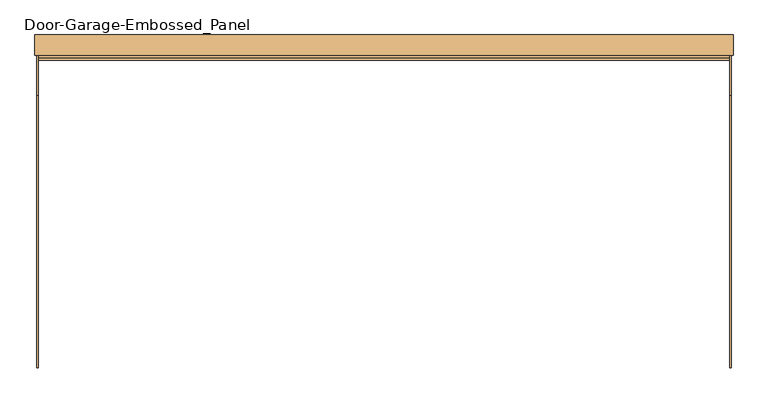
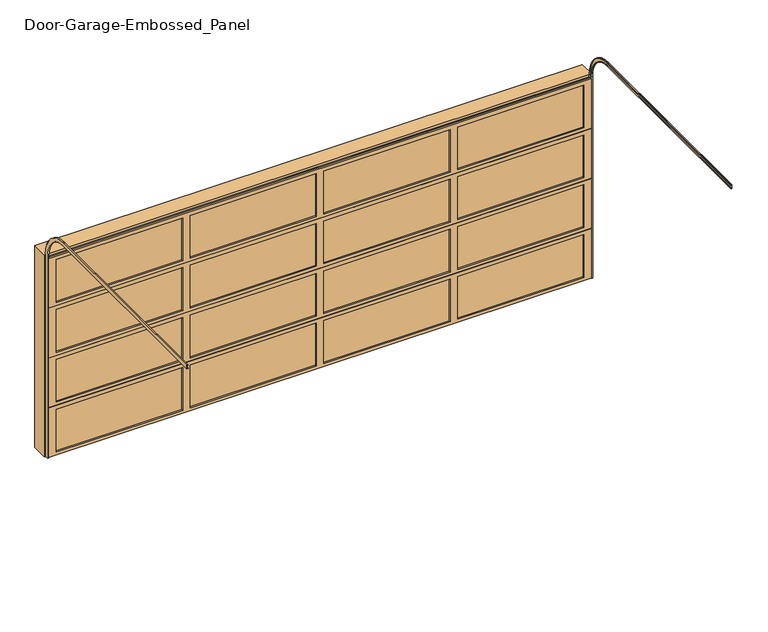
"""IFC4 building model written with IfcOpenShell, lengths in millimetres: door geometry, Door-Garage-Embossed_Panel : 216'' x 84''."""

from ifc_helpers import new_model, si_unit, frame, origin, place, context, project, spatial, polyline, circle_curve, outline, extrude, faceted_brep, source, transform, mapped, element, save
from ifc_brep_helpers import plane_surface, cylinder_surface, revolved_surface, advanced_brep


def door_garage_embossed_panel_c404131a(model_context):
    return source(origin(), model_context, "Body", "SolidModel", [
        extrude(outline(polyline([(1314.45, -100.0125), (1314.45, -106.3625), (38.1, -106.3625), (38.1, -100.0125), (1314.45, -100.0125)])), frame((0.0, 0.0, 1638.3), z_axis=(0.0, 0.0, 1.0), x_axis=(1.0, 0.0, 0.0)), (0.0, 0.0, 1.0), 457.2),
        extrude(outline(polyline([(-38.1, -100.0125), (-38.1, -106.3625), (-1314.45, -106.3625), (-1314.45, -100.0125), (-38.1, -100.0125)])), frame((0.0, 0.0, 1638.3), z_axis=(0.0, 0.0, 1.0), x_axis=(1.0, 0.0, 0.0)), (0.0, 0.0, 1.0), 457.2),
        extrude(outline(polyline([(2667.0, -100.0125), (2667.0, -106.3625), (1390.65, -106.3625), (1390.65, -100.0125), (2667.0, -100.0125)])), frame((0.0, 0.0, 1638.3), z_axis=(0.0, 0.0, 1.0), x_axis=(1.0, 0.0, 0.0)), (0.0, 0.0, 1.0), 457.2),
        extrude(outline(polyline([(-1390.65, -100.0125), (-1390.65, -106.3625), (-2667.0, -106.3625), (-2667.0, -100.0125), (-1390.65, -100.0125)])), frame((0.0, 0.0, 1638.3), z_axis=(0.0, 0.0, 1.0), x_axis=(1.0, 0.0, 0.0)), (0.0, 0.0, 1.0), 457.2),
        faceted_brep([(2743.2, -106.3625, 2136.775), (2743.2, -122.2375, 2136.775), (2743.2, -122.2375, 1606.55), (2743.2, -100.0125, 1606.55), (2743.2, -100.0125, 1600.2), (2743.2, -84.1375, 1600.2), (2743.2, -84.1375, 2130.425), (2743.2, -106.3625, 2130.425), (-2743.2, -122.2375, 2136.775), (-2743.2, -106.3625, 2136.775), (-2743.2, -106.3625, 2130.425), (-2743.2, -84.1375, 2130.425), (-2743.2, -84.1375, 1600.2), (-2743.2, -100.0125, 1600.2), (-2743.2, -100.0125, 1606.55), (-2743.2, -122.2375, 1606.55), (1390.65, -122.2375, 2095.5), (2667.0, -122.2375, 2095.5), (2667.0, -122.2375, 1638.3), (1390.65, -122.2375, 1638.3), (-1314.45, -122.2375, 2095.5), (-38.1, -122.2375, 2095.5), (-38.1, -122.2375, 1638.3), (-1314.45, -122.2375, 1638.3), (38.1, -122.2375, 2095.5), (1314.45, -122.2375, 2095.5), (1314.45, -122.2375, 1638.3), (38.1, -122.2375, 1638.3), (-2667.0, -122.2375, 2095.5), (-1390.65, -122.2375, 2095.5), (-1390.65, -122.2375, 1638.3), (-2667.0, -122.2375, 1638.3), (2667.0, -84.1375, 2095.5), (1390.65, -84.1375, 2095.5), (1390.65, -84.1375, 1638.3), (2667.0, -84.1375, 1638.3), (-38.1, -84.1375, 2095.5), (-1314.45, -84.1375, 2095.5), (-1314.45, -84.1375, 1638.3), (-38.1, -84.1375, 1638.3), (1314.45, -84.1375, 2095.5), (38.1, -84.1375, 2095.5), (38.1, -84.1375, 1638.3), (1314.45, -84.1375, 1638.3), (-1390.65, -84.1375, 2095.5), (-2667.0, -84.1375, 2095.5), (-2667.0, -84.1375, 1638.3), (-1390.65, -84.1375, 1638.3)], [[[0, 1, 2, 3, 4, 5, 6, 7]], [[8, 9, 10, 11, 12, 13, 14, 15]], [[1, 0, 9, 8]], [[2, 1, 8, 15], [16, 17, 18, 19], [20, 21, 22, 23], [24, 25, 26, 27], [28, 29, 30, 31]], [[3, 2, 15, 14]], [[4, 3, 14, 13]], [[5, 4, 13, 12]], [[6, 5, 12, 11], [32, 33, 34, 35], [36, 37, 38, 39], [40, 41, 42, 43], [44, 45, 46, 47]], [[7, 6, 11, 10]], [[0, 7, 10, 9]], [[16, 33, 32, 17]], [[33, 16, 19, 34]], [[34, 19, 18, 35]], [[17, 32, 35, 18]], [[20, 37, 36, 21]], [[37, 20, 23, 38]], [[38, 23, 22, 39]], [[21, 36, 39, 22]], [[24, 41, 40, 25]], [[41, 24, 27, 42]], [[42, 27, 26, 43]], [[25, 40, 43, 26]], [[28, 45, 44, 29]], [[45, 28, 31, 46]], [[46, 31, 30, 47]], [[29, 44, 47, 30]]]),
        extrude(outline(polyline([(1314.45, -100.0125), (1314.45, -106.3625), (38.1, -106.3625), (38.1, -100.0125), (1314.45, -100.0125)])), frame((0.0, 0.0, 1104.9), z_axis=(0.0, 0.0, 1.0), x_axis=(1.0, 0.0, 0.0)), (0.0, 0.0, 1.0), 457.2),
        extrude(outline(polyline([(-38.1, -100.0125), (-38.1, -106.3625), (-1314.45, -106.3625), (-1314.45, -100.0125), (-38.1, -100.0125)])), frame((0.0, 0.0, 1104.9), z_axis=(0.0, 0.0, 1.0), x_axis=(1.0, 0.0, 0.0)), (0.0, 0.0, 1.0), 457.2),
        extrude(outline(polyline([(2667.0, -100.0125), (2667.0, -106.3625), (1390.65, -106.3625), (1390.65, -100.0125), (2667.0, -100.0125)])), frame((0.0, 0.0, 1104.9), z_axis=(0.0, 0.0, 1.0), x_axis=(1.0, 0.0, 0.0)), (0.0, 0.0, 1.0), 457.2),
        extrude(outline(polyline([(-1390.65, -100.0125), (-1390.65, -106.3625), (-2667.0, -106.3625), (-2667.0, -100.0125), (-1390.65, -100.0125)])), frame((0.0, 0.0, 1104.9), z_axis=(0.0, 0.0, 1.0), x_axis=(1.0, 0.0, 0.0)), (0.0, 0.0, 1.0), 457.2),
        faceted_brep([(2743.2, -106.3625, 1603.375), (2743.2, -122.2375, 1603.375), (2743.2, -122.2375, 1073.15), (2743.2, -100.0125, 1073.15), (2743.2, -100.0125, 1066.8), (2743.2, -84.1375, 1066.8), (2743.2, -84.1375, 1597.025), (2743.2, -106.3625, 1597.025), (-2743.2, -122.2375, 1603.375), (-2743.2, -106.3625, 1603.375), (-2743.2, -106.3625, 1597.025), (-2743.2, -84.1375, 1597.025), (-2743.2, -84.1375, 1066.8), (-2743.2, -100.0125, 1066.8), (-2743.2, -100.0125, 1073.15), (-2743.2, -122.2375, 1073.15), (1390.65, -122.2375, 1562.1), (2667.0, -122.2375, 1562.1), (2667.0, -122.2375, 1104.9), (1390.65, -122.2375, 1104.9), (-1314.45, -122.2375, 1562.1), (-38.1, -122.2375, 1562.1), (-38.1, -122.2375, 1104.9), (-1314.45, -122.2375, 1104.9), (38.1, -122.2375, 1562.1), (1314.45, -122.2375, 1562.1), (1314.45, -122.2375, 1104.9), (38.1, -122.2375, 1104.9), (-2667.0, -122.2375, 1562.1), (-1390.65, -122.2375, 1562.1), (-1390.65, -122.2375, 1104.9), (-2667.0, -122.2375, 1104.9), (2667.0, -84.1375, 1562.1), (1390.65, -84.1375, 1562.1), (1390.65, -84.1375, 1104.9), (2667.0, -84.1375, 1104.9), (-38.1, -84.1375, 1562.1), (-1314.45, -84.1375, 1562.1), (-1314.45, -84.1375, 1104.9), (-38.1, -84.1375, 1104.9), (1314.45, -84.1375, 1562.1), (38.1, -84.1375, 1562.1), (38.1, -84.1375, 1104.9), (1314.45, -84.1375, 1104.9), (-1390.65, -84.1375, 1562.1), (-2667.0, -84.1375, 1562.1), (-2667.0, -84.1375, 1104.9), (-1390.65, -84.1375, 1104.9)], [[[0, 1, 2, 3, 4, 5, 6, 7]], [[8, 9, 10, 11, 12, 13, 14, 15]], [[1, 0, 9, 8]], [[2, 1, 8, 15], [16, 17, 18, 19], [20, 21, 22, 23], [24, 25, 26, 27], [28, 29, 30, 31]], [[3, 2, 15, 14]], [[4, 3, 14, 13]], [[5, 4, 13, 12]], [[6, 5, 12, 11], [32, 33, 34, 35], [36, 37, 38, 39], [40, 41, 42, 43], [44, 45, 46, 47]], [[7, 6, 11, 10]], [[0, 7, 10, 9]], [[16, 33, 32, 17]], [[33, 16, 19, 34]], [[34, 19, 18, 35]], [[17, 32, 35, 18]], [[20, 37, 36, 21]], [[37, 20, 23, 38]], [[38, 23, 22, 39]], [[21, 36, 39, 22]], [[24, 41, 40, 25]], [[41, 24, 27, 42]], [[42, 27, 26, 43]], [[25, 40, 43, 26]], [[28, 45, 44, 29]], [[45, 28, 31, 46]], [[46, 31, 30, 47]], [[29, 44, 47, 30]]]),
        extrude(outline(polyline([(1314.45, -100.0125), (1314.45, -106.3625), (38.1, -106.3625), (38.1, -100.0125), (1314.45, -100.0125)])), frame((0.0, 0.0, 571.5), z_axis=(0.0, 0.0, 1.0), x_axis=(1.0, 0.0, 0.0)), (0.0, 0.0, 1.0), 457.2),
        extrude(outline(polyline([(-38.1, -100.0125), (-38.1, -106.3625), (-1314.45, -106.3625), (-1314.45, -100.0125), (-38.1, -100.0125)])), frame((0.0, 0.0, 571.5), z_axis=(0.0, 0.0, 1.0), x_axis=(1.0, 0.0, 0.0)), (0.0, 0.0, 1.0), 457.2),
        extrude(outline(polyline([(2667.0, -100.0125), (2667.0, -106.3625), (1390.65, -106.3625), (1390.65, -100.0125), (2667.0, -100.0125)])), frame((0.0, 0.0, 571.5), z_axis=(0.0, 0.0, 1.0), x_axis=(1.0, 0.0, 0.0)), (0.0, 0.0, 1.0), 457.2),
        extrude(outline(polyline([(-1390.65, -100.0125), (-1390.65, -106.3625), (-2667.0, -106.3625), (-2667.0, -100.0125), (-1390.65, -100.0125)])), frame((0.0, 0.0, 571.5), z_axis=(0.0, 0.0, 1.0), x_axis=(1.0, 0.0, 0.0)), (0.0, 0.0, 1.0), 457.2),
        faceted_brep([(2743.2, -106.3625, 1069.975), (2743.2, -122.2375, 1069.975), (2743.2, -122.2375, 539.75), (2743.2, -100.0125, 539.75), (2743.2, -100.0125, 533.4), (2743.2, -84.1375, 533.4), (2743.2, -84.1375, 1063.625), (2743.2, -106.3625, 1063.625), (-2743.2, -122.2375, 1069.975), (-2743.2, -106.3625, 1069.975), (-2743.2, -106.3625, 1063.625), (-2743.2, -84.1375, 1063.625), (-2743.2, -84.1375, 533.4), (-2743.2, -100.0125, 533.4), (-2743.2, -100.0125, 539.75), (-2743.2, -122.2375, 539.75), (1390.65, -122.2375, 1028.7), (2667.0, -122.2375, 1028.7), (2667.0, -122.2375, 571.5), (1390.65, -122.2375, 571.5), (-1314.45, -122.2375, 1028.7), (-38.1, -122.2375, 1028.7), (-38.1, -122.2375, 571.5), (-1314.45, -122.2375, 571.5), (38.1, -122.2375, 1028.7), (1314.45, -122.2375, 1028.7), (1314.45, -122.2375, 571.5), (38.1, -122.2375, 571.5), (-2667.0, -122.2375, 1028.7), (-1390.65, -122.2375, 1028.7), (-1390.65, -122.2375, 571.5), (-2667.0, -122.2375, 571.5), (2667.0, -84.1375, 1028.7), (1390.65, -84.1375, 1028.7), (1390.65, -84.1375, 571.5), (2667.0, -84.1375, 571.5), (-38.1, -84.1375, 1028.7), (-1314.45, -84.1375, 1028.7), (-1314.45, -84.1375, 571.5), (-38.1, -84.1375, 571.5), (1314.45, -84.1375, 1028.7), (38.1, -84.1375, 1028.7), (38.1, -84.1375, 571.5), (1314.45, -84.1375, 571.5), (-1390.65, -84.1375, 1028.7), (-2667.0, -84.1375, 1028.7), (-2667.0, -84.1375, 571.5), (-1390.65, -84.1375, 571.5)], [[[0, 1, 2, 3, 4, 5, 6, 7]], [[8, 9, 10, 11, 12, 13, 14, 15]], [[1, 0, 9, 8]], [[2, 1, 8, 15], [16, 17, 18, 19], [20, 21, 22, 23], [24, 25, 26, 27], [28, 29, 30, 31]], [[3, 2, 15, 14]], [[4, 3, 14, 13]], [[5, 4, 13, 12]], [[6, 5, 12, 11], [32, 33, 34, 35], [36, 37, 38, 39], [40, 41, 42, 43], [44, 45, 46, 47]], [[7, 6, 11, 10]], [[0, 7, 10, 9]], [[16, 33, 32, 17]], [[33, 16, 19, 34]], [[34, 19, 18, 35]], [[17, 32, 35, 18]], [[20, 37, 36, 21]], [[37, 20, 23, 38]], [[38, 23, 22, 39]], [[21, 36, 39, 22]], [[24, 41, 40, 25]], [[41, 24, 27, 42]], [[42, 27, 26, 43]], [[25, 40, 43, 26]], [[28, 45, 44, 29]], [[45, 28, 31, 46]], [[46, 31, 30, 47]], [[29, 44, 47, 30]]]),
        extrude(outline(polyline([(1314.45, -100.0125), (1314.45, -106.3625), (38.1, -106.3625), (38.1, -100.0125), (1314.45, -100.0125)])), frame((0.0, 0.0, 38.1), z_axis=(0.0, 0.0, 1.0), x_axis=(1.0, 0.0, 0.0)), (0.0, 0.0, 1.0), 457.2),
        extrude(outline(polyline([(-38.1, -100.0125), (-38.1, -106.3625), (-1314.45, -106.3625), (-1314.45, -100.0125), (-38.1, -100.0125)])), frame((0.0, 0.0, 38.1), z_axis=(0.0, 0.0, 1.0), x_axis=(1.0, 0.0, 0.0)), (0.0, 0.0, 1.0), 457.2),
        extrude(outline(polyline([(2667.0, -100.0125), (2667.0, -106.3625), (1390.65, -106.3625), (1390.65, -100.0125), (2667.0, -100.0125)])), frame((0.0, 0.0, 38.1), z_axis=(0.0, 0.0, 1.0), x_axis=(1.0, 0.0, 0.0)), (0.0, 0.0, 1.0), 457.2),
        extrude(outline(polyline([(-1390.65, -100.0125), (-1390.65, -106.3625), (-2667.0, -106.3625), (-2667.0, -100.0125), (-1390.65, -100.0125)])), frame((0.0, 0.0, 38.1), z_axis=(0.0, 0.0, 1.0), x_axis=(1.0, 0.0, 0.0)), (0.0, 0.0, 1.0), 457.2),
        faceted_brep([(2743.2, -106.3625, 536.575), (2743.2, -122.2375, 536.575), (2743.2, -122.2375, 6.35), (2743.2, -100.0125, 6.35), (2743.2, -100.0125, 0.0), (2743.2, -84.1375, 0.0), (2743.2, -84.1375, 530.225), (2743.2, -106.3625, 530.225), (-2743.2, -122.2375, 536.575), (-2743.2, -106.3625, 536.575), (-2743.2, -106.3625, 530.225), (-2743.2, -84.1375, 530.225), (-2743.2, -84.1375, 0.0), (-2743.2, -100.0125, 0.0), (-2743.2, -100.0125, 6.35), (-2743.2, -122.2375, 6.35), (1390.65, -122.2375, 495.3), (2667.0, -122.2375, 495.3), (2667.0, -122.2375, 38.1), (1390.65, -122.2375, 38.1), (-1314.45, -122.2375, 495.3), (-38.1, -122.2375, 495.3), (-38.1, -122.2375, 38.1), (-1314.45, -122.2375, 38.1), (38.1, -122.2375, 495.3), (1314.45, -122.2375, 495.3), (1314.45, -122.2375, 38.1), (38.1, -122.2375, 38.1), (-2667.0, -122.2375, 495.3), (-1390.65, -122.2375, 495.3), (-1390.65, -122.2375, 38.1), (-2667.0, -122.2375, 38.1), (2667.0, -84.1375, 495.3), (1390.65, -84.1375, 495.3), (1390.65, -84.1375, 38.1), (2667.0, -84.1375, 38.1), (-38.1, -84.1375, 495.3), (-1314.45, -84.1375, 495.3), (-1314.45, -84.1375, 38.1), (-38.1, -84.1375, 38.1), (1314.45, -84.1375, 495.3), (38.1, -84.1375, 495.3), (38.1, -84.1375, 38.1), (1314.45, -84.1375, 38.1), (-1390.65, -84.1375, 495.3), (-2667.0, -84.1375, 495.3), (-2667.0, -84.1375, 38.1), (-1390.65, -84.1375, 38.1)], [[[0, 1, 2, 3, 4, 5, 6, 7]], [[8, 9, 10, 11, 12, 13, 14, 15]], [[1, 0, 9, 8]], [[2, 1, 8, 15], [16, 17, 18, 19], [20, 21, 22, 23], [24, 25, 26, 27], [28, 29, 30, 31]], [[3, 2, 15, 14]], [[4, 3, 14, 13]], [[5, 4, 13, 12]], [[6, 5, 12, 11], [32, 33, 34, 35], [36, 37, 38, 39], [40, 41, 42, 43], [44, 45, 46, 47]], [[7, 6, 11, 10]], [[0, 7, 10, 9]], [[16, 33, 32, 17]], [[33, 16, 19, 34]], [[34, 19, 18, 35]], [[17, 32, 35, 18]], [[20, 37, 36, 21]], [[37, 20, 23, 38]], [[38, 23, 22, 39]], [[21, 36, 39, 22]], [[24, 41, 40, 25]], [[41, 24, 27, 42]], [[42, 27, 26, 43]], [[25, 40, 43, 26]], [[28, 45, 44, 29]], [[45, 28, 31, 46]], [[46, 31, 30, 47]], [[29, 44, 47, 30]]]),
        advanced_brep(
        [(2755.9, -122.2375, 0.0), (2743.2, -122.2375, 0.0), (2743.2, -119.0625, 0.0), (2752.725, -119.0625, 0.0), (2752.725, -87.3125, 0.0), (2743.2, -87.3125, 0.0), (2743.2, -84.1375, 0.0), (2755.9, -84.1375, 0.0), (2755.9, -122.2375, 2159.0), (2743.2, -122.2375, 2159.0), (2743.2, -401.6375, 2438.4), (2743.2, -2560.6375, 2438.4), (2743.2, -2560.6375, 2441.575), (2743.2, -401.6375, 2441.575), (2743.2, -119.0625, 2159.0), (2752.725, -119.0625, 2159.0), (2752.725, -401.6375, 2441.575), (2752.725, -2560.6375, 2441.575), (2752.725, -2560.6375, 2473.325), (2752.725, -401.6375, 2473.325), (2752.725, -87.3125, 2159.0), (2743.2, -87.3125, 2159.0), (2743.2, -401.6375, 2473.325), (2743.2, -2560.6375, 2473.325), (2743.2, -2560.6375, 2476.5), (2743.2, -401.6375, 2476.5), (2743.2, -84.1375, 2159.0), (2755.9, -84.1375, 2159.0), (2755.9, -401.6375, 2476.5), (2755.9, -2560.6375, 2476.5), (2755.9, -2560.6375, 2438.4), (2755.9, -401.6375, 2438.4)],
        [
            (0, 1),
            (1, 2),
            (2, 3),
            (3, 4),
            (4, 5),
            (5, 6),
            (6, 7),
            (7, 0),
            (0, 8),
            (8, 9),
            (9, 1),
            (9, 10, circle_curve(frame((2743.2, -401.6375, 2159.0), z_axis=(1.0, 0.0, 0.0), x_axis=(0.0, 1.0, 0.0)), 279.4)),
            (10, 11),
            (11, 12),
            (12, 13),
            (13, 14, circle_curve(frame((2743.2, -401.6375, 2159.0), z_axis=(-1.0, 0.0, 0.0), x_axis=(0.0, 1.0, 0.0)), 282.575)),
            (14, 2),
            (14, 15),
            (15, 3),
            (15, 16, circle_curve(frame((2752.725, -401.6375, 2159.0), z_axis=(1.0, 0.0, 0.0), x_axis=(0.0, 1.0, 0.0)), 282.575)),
            (16, 17),
            (17, 18),
            (18, 19),
            (19, 20, circle_curve(frame((2752.725, -401.6375, 2159.0), z_axis=(-1.0, 0.0, 0.0), x_axis=(0.0, 1.0, 0.0)), 314.325)),
            (20, 4),
            (20, 21),
            (21, 5),
            (21, 22, circle_curve(frame((2743.2, -401.6375, 2159.0), z_axis=(1.0, 0.0, 0.0), x_axis=(0.0, 1.0, 0.0)), 314.325)),
            (22, 23),
            (23, 24),
            (24, 25),
            (25, 26, circle_curve(frame((2743.2, -401.6375, 2159.0), z_axis=(-1.0, 0.0, 0.0), x_axis=(0.0, 1.0, 0.0)), 317.5)),
            (26, 6),
            (26, 27),
            (27, 7),
            (27, 28, circle_curve(frame((2755.9, -401.6375, 2159.0), z_axis=(1.0, 0.0, 0.0), x_axis=(0.0, 1.0, 0.0)), 317.5)),
            (28, 29),
            (29, 30),
            (30, 31),
            (31, 8, circle_curve(frame((2755.9, -401.6375, 2159.0), z_axis=(-1.0, 0.0, 0.0), x_axis=(0.0, 1.0, 0.0)), 279.4)),
            (31, 10),
            (13, 16),
            (19, 22),
            (25, 28),
            (29, 24),
            (23, 18),
            (17, 12),
            (11, 30),
        ],
        [
            plane_surface(frame((0.0, -122.2375, 0.0), z_axis=(0.0, 0.0, -1.0), x_axis=(1.0, 0.0, 0.0))),
            plane_surface(frame((2755.9, -122.2375, 0.0), z_axis=(0.0, -1.0, 0.0), x_axis=(0.0, 0.0, 1.0))),
            plane_surface(frame((2743.2, -122.2375, 0.0), z_axis=(-1.0, 0.0, 0.0), x_axis=(0.0, 0.0, 1.0))),
            plane_surface(frame((2743.2, -119.0625, 0.0), z_axis=(0.0, 1.0, 0.0), x_axis=(0.0, 0.0, 1.0))),
            plane_surface(frame((2752.725, -119.0625, 0.0), z_axis=(-1.0, 0.0, 0.0), x_axis=(0.0, 0.0, 1.0))),
            plane_surface(frame((2752.725, -87.3125, 0.0), z_axis=(0.0, -1.0, 0.0), x_axis=(0.0, 0.0, 1.0))),
            plane_surface(frame((2743.2, -87.3125, 0.0), z_axis=(-1.0, 0.0, 0.0), x_axis=(0.0, 0.0, 1.0))),
            plane_surface(frame((2743.2, -84.1375, 0.0), z_axis=(0.0, 1.0, 0.0), x_axis=(0.0, 0.0, 1.0))),
            plane_surface(frame((2755.9, -84.1375, 0.0), z_axis=(1.0, 0.0, 0.0), x_axis=(0.0, 0.0, 1.0))),
            revolved_surface(polyline([(2755.9, -122.23750000000001, 2159.0), (2743.2, -122.23750000000001, 2159.0)]), (0.0, -401.6375, 2159.0), (1.0, 0.0, 0.0)),
            cylinder_surface(frame((0.0, -401.6375, 2159.0), z_axis=(1.0, 0.0, 0.0), x_axis=(0.0, 1.0, 0.0)), 282.575),
            revolved_surface(polyline([(2752.725, -87.3125, 2159.0), (2743.2, -87.3125, 2159.0)]), (0.0, -401.6375, 2159.0), (1.0, 0.0, 0.0)),
            cylinder_surface(frame((0.0, -401.6375, 2159.0), z_axis=(1.0, 0.0, 0.0), x_axis=(0.0, 1.0, 0.0)), 317.5),
            plane_surface(frame((0.0, -2560.6375, 2438.4), z_axis=(0.0, -1.0, 0.0), x_axis=(1.0, 0.0, 0.0))),
            plane_surface(frame((2755.9, -401.6375, 2438.4), z_axis=(0.0, 0.0, -1.0), x_axis=(0.0, -1.0, 0.0))),
            plane_surface(frame((2743.2, -401.6375, 2441.575), z_axis=(0.0, 0.0, 1.0), x_axis=(0.0, -1.0, 0.0))),
            plane_surface(frame((2752.725, -401.6375, 2473.325), z_axis=(0.0, 0.0, -1.0), x_axis=(0.0, -1.0, 0.0))),
            plane_surface(frame((2743.2, -401.6375, 2476.5), z_axis=(0.0, 0.0, 1.0), x_axis=(0.0, -1.0, 0.0))),
        ],
        [
            (0, [[1, 2, 3, 4, 5, 6, 7, 8]]),
            (1, [[-1, 9, 10, 11]]),
            (2, [[-2, -11, 12, 13, 14, 15, 16, 17]]),
            (3, [[-3, -17, 18, 19]]),
            (4, [[-4, -19, 20, 21, 22, 23, 24, 25]]),
            (5, [[-5, -25, 26, 27]]),
            (6, [[-6, -27, 28, 29, 30, 31, 32, 33]]),
            (7, [[-7, -33, 34, 35]]),
            (8, [[-8, -35, 36, 37, 38, 39, 40, -9]]),
            (9, [[-12, -10, -40, 41]]),
            (10, [[-20, -18, -16, 42]]),
            (11, [[-28, -26, -24, 43]]),
            (12, [[-36, -34, -32, 44]]),
            (13, [[-38, 45, -30, 46, -22, 47, -14, 48]]),
            (14, [[-41, -39, -48, -13]]),
            (15, [[-42, -15, -47, -21]]),
            (16, [[-43, -23, -46, -29]]),
            (17, [[-44, -31, -45, -37]]),
        ],
    ),
        advanced_brep(
        [(-2755.9, -122.2375, 0.0), (-2755.9, -84.1375, 0.0), (-2743.2, -84.1375, 0.0), (-2743.2, -87.3125, 0.0), (-2752.725, -87.3125, 0.0), (-2752.725, -119.0625, 0.0), (-2743.2, -119.0625, 0.0), (-2743.2, -122.2375, 0.0), (-2755.9, -122.2375, 2159.0), (-2755.9, -401.6375, 2438.4), (-2755.9, -2560.6375, 2438.4), (-2755.9, -2560.6375, 2476.5), (-2755.9, -401.6375, 2476.5), (-2755.9, -84.1375, 2159.0), (-2743.2, -84.1375, 2159.0), (-2743.2, -401.6375, 2476.5), (-2743.2, -2560.6375, 2476.5), (-2743.2, -2560.6375, 2473.325), (-2743.2, -401.6375, 2473.325), (-2743.2, -87.3125, 2159.0), (-2752.725, -87.3125, 2159.0), (-2752.725, -401.6375, 2473.325), (-2752.725, -2560.6375, 2473.325), (-2752.725, -2560.6375, 2441.575), (-2752.725, -401.6375, 2441.575), (-2752.725, -119.0625, 2159.0), (-2743.2, -119.0625, 2159.0), (-2743.2, -401.6375, 2441.575), (-2743.2, -2560.6375, 2441.575), (-2743.2, -2560.6375, 2438.4), (-2743.2, -401.6375, 2438.4), (-2743.2, -122.2375, 2159.0)],
        [
            (0, 1),
            (1, 2),
            (2, 3),
            (3, 4),
            (4, 5),
            (5, 6),
            (6, 7),
            (7, 0),
            (0, 8),
            (8, 9, circle_curve(frame((-2755.9, -401.6375, 2159.0), z_axis=(1.0, 0.0, 0.0), x_axis=(0.0, 1.0, 0.0)), 279.4)),
            (9, 10),
            (10, 11),
            (11, 12),
            (12, 13, circle_curve(frame((-2755.9, -401.6375, 2159.0), z_axis=(-1.0, 0.0, 0.0), x_axis=(0.0, 1.0, 0.0)), 317.5)),
            (13, 1),
            (13, 14),
            (14, 2),
            (14, 15, circle_curve(frame((-2743.2, -401.6375, 2159.0), z_axis=(1.0, 0.0, 0.0), x_axis=(0.0, 1.0, 0.0)), 317.5)),
            (15, 16),
            (16, 17),
            (17, 18),
            (18, 19, circle_curve(frame((-2743.2, -401.6375, 2159.0), z_axis=(-1.0, 0.0, 0.0), x_axis=(0.0, 1.0, 0.0)), 314.325)),
            (19, 3),
            (19, 20),
            (20, 4),
            (20, 21, circle_curve(frame((-2752.725, -401.6375, 2159.0), z_axis=(1.0, 0.0, 0.0), x_axis=(0.0, 1.0, 0.0)), 314.325)),
            (21, 22),
            (22, 23),
            (23, 24),
            (24, 25, circle_curve(frame((-2752.725, -401.6375, 2159.0), z_axis=(-1.0, 0.0, 0.0), x_axis=(0.0, 1.0, 0.0)), 282.575)),
            (25, 5),
            (25, 26),
            (26, 6),
            (26, 27, circle_curve(frame((-2743.2, -401.6375, 2159.0), z_axis=(1.0, 0.0, 0.0), x_axis=(0.0, 1.0, 0.0)), 282.575)),
            (27, 28),
            (28, 29),
            (29, 30),
            (30, 31, circle_curve(frame((-2743.2, -401.6375, 2159.0), z_axis=(-1.0, 0.0, 0.0), x_axis=(0.0, 1.0, 0.0)), 279.4)),
            (31, 7),
            (31, 8),
            (12, 15),
            (18, 21),
            (24, 27),
            (30, 9),
            (10, 29),
            (28, 23),
            (22, 17),
            (16, 11),
        ],
        [
            plane_surface(frame((0.0, -122.2375, 0.0), z_axis=(0.0, 0.0, -1.0), x_axis=(1.0, 0.0, 0.0))),
            plane_surface(frame((-2755.9, -122.2375, 0.0), z_axis=(-1.0, 0.0, 0.0), x_axis=(0.0, 0.0, 1.0))),
            plane_surface(frame((-2755.9, -84.1375, 0.0), z_axis=(0.0, 1.0, 0.0), x_axis=(0.0, 0.0, 1.0))),
            plane_surface(frame((-2743.2, -84.1375, 0.0), z_axis=(1.0, 0.0, 0.0), x_axis=(0.0, 0.0, 1.0))),
            plane_surface(frame((-2743.2, -87.3125, 0.0), z_axis=(0.0, -1.0, 0.0), x_axis=(0.0, 0.0, 1.0))),
            plane_surface(frame((-2752.725, -87.3125, 0.0), z_axis=(1.0, 0.0, 0.0), x_axis=(0.0, 0.0, 1.0))),
            plane_surface(frame((-2752.725, -119.0625, 0.0), z_axis=(0.0, 1.0, 0.0), x_axis=(0.0, 0.0, 1.0))),
            plane_surface(frame((-2743.2, -119.0625, 0.0), z_axis=(1.0, 0.0, 0.0), x_axis=(0.0, 0.0, 1.0))),
            plane_surface(frame((-2743.2, -122.2375, 0.0), z_axis=(0.0, -1.0, 0.0), x_axis=(0.0, 0.0, 1.0))),
            cylinder_surface(frame((0.0, -401.6375, 2159.0), z_axis=(1.0, 0.0, 0.0), x_axis=(0.0, 1.0, 0.0)), 317.5),
            revolved_surface(polyline([(-2743.2, -87.3125, 2159.0), (-2752.725, -87.3125, 2159.0)]), (0.0, -401.6375, 2159.0), (1.0, 0.0, 0.0)),
            cylinder_surface(frame((0.0, -401.6375, 2159.0), z_axis=(1.0, 0.0, 0.0), x_axis=(0.0, 1.0, 0.0)), 282.575),
            revolved_surface(polyline([(-2743.2, -122.23750000000001, 2159.0), (-2755.9, -122.23750000000001, 2159.0)]), (0.0, -401.6375, 2159.0), (1.0, 0.0, 0.0)),
            plane_surface(frame((0.0, -2560.6375, 2438.4), z_axis=(0.0, -1.0, 0.0), x_axis=(1.0, 0.0, 0.0))),
            plane_surface(frame((-2755.9, -401.6375, 2476.5), z_axis=(0.0, 0.0, 1.0), x_axis=(0.0, -1.0, 0.0))),
            plane_surface(frame((-2743.2, -401.6375, 2473.325), z_axis=(0.0, 0.0, -1.0), x_axis=(0.0, -1.0, 0.0))),
            plane_surface(frame((-2752.725, -401.6375, 2441.575), z_axis=(0.0, 0.0, 1.0), x_axis=(0.0, -1.0, 0.0))),
            plane_surface(frame((-2743.2, -401.6375, 2438.4), z_axis=(0.0, 0.0, -1.0), x_axis=(0.0, -1.0, 0.0))),
        ],
        [
            (0, [[1, 2, 3, 4, 5, 6, 7, 8]]),
            (1, [[-1, 9, 10, 11, 12, 13, 14, 15]]),
            (2, [[-2, -15, 16, 17]]),
            (3, [[-3, -17, 18, 19, 20, 21, 22, 23]]),
            (4, [[-4, -23, 24, 25]]),
            (5, [[-5, -25, 26, 27, 28, 29, 30, 31]]),
            (6, [[-6, -31, 32, 33]]),
            (7, [[-7, -33, 34, 35, 36, 37, 38, 39]]),
            (8, [[-8, -39, 40, -9]]),
            (9, [[-18, -16, -14, 41]]),
            (10, [[-26, -24, -22, 42]]),
            (11, [[-34, -32, -30, 43]]),
            (12, [[-10, -40, -38, 44]]),
            (13, [[45, -36, 46, -28, 47, -20, 48, -12]]),
            (14, [[-41, -13, -48, -19]]),
            (15, [[-42, -21, -47, -27]]),
            (16, [[-43, -29, -46, -35]]),
            (17, [[-44, -37, -45, -11]]),
        ],
    ),
        extrude(outline(polyline([(0.0, 2743.2), (0.0, 2768.6), (2159.0, 2768.6), (2159.0, -2768.6), (0.0, -2768.6), (0.0, -2743.2), (2133.6, -2743.2), (2133.6, 2743.2), (0.0, 2743.2)])), frame((0.0, -84.1375, 0.0), z_axis=(0.0, 1.0, 0.0), x_axis=(0.0, 0.0, 1.0)), (0.0, 0.0, 1.0), 161.925),
    ])


if __name__ == "__main__":
    model = new_model("IFC4")
    model_context = context("Model", 3, world=origin())
    ifc_project = project(units=[si_unit("LENGTHUNIT", "METRE", prefix="MILLI")], contexts=[model_context])
    site = spatial("IfcSite", under=ifc_project)
    building = spatial("IfcBuilding", under=site)
    placement = place(None, origin())
    door_garage_embossed_panel_shape = door_garage_embossed_panel_c404131a(model_context)
    element("IfcDoor", 1, ObjectType="Door-Garage-Embossed_Panel : 216'' x 84''", at=placement, inside=building, context=model_context, shape_type="MappedRepresentation", body=[
        mapped(door_garage_embossed_panel_shape, transform((0.0, 0.0, 0.0), x_axis=(1.0, 0.0, 0.0), y_axis=(0.0, 1.0, 0.0), z_axis=(0.0, 0.0, 1.0))),
    ])
    save(model, "model.ifc")

# Revit data of these elements
# Type "Door-Garage-Embossed_Panel : 216'' x 84''"
#   Type Mark = "82"
#   COBie.Type.CreatedBy = "info@geappliances.com"
#   COBie.Type.CreatedOn = "2017-07-20T03:49:29"
#   COBie.Type.Name = "Door-Garage-Embossed_Panel_216'' x 84''_82"
#   COBie.Type.Category = "23-30 10 00 : Doors"
#   COBie.Type.Description = "Door-Garage-Embossed_Panel_216'' x 84''"
#   COBie.Type.Manufacturer = ""
#   COBie.Type.ModelNumber = ""
#   Analytic Construction = "Wooden"
#   COBie.Type.ReplacementCost = 0
#   Thickness = 0' - 1 1/2"
#   Thermal Resistance (R) = 0.455703 (m²·K)/W
#   Rough Width = 18' - 2"
#   Rough Height = 7' - 1"
#   Panel Height = 1' - 9"
#   Height = 7' - 0"
#   Width = 18' - 0"
#   Heat Transfer Coefficient (U) = 2.19465 W/(m²·K)
#   COBie.Type = yes
#   Panels = 4
#   Function = 1
#   Exterior Trim [instance default] = yes
#   Trim Material = Trim - White
#   Panel Material = Trim - White
#   Frame Material = Trim - White
#   Visual Light Transmittance = 0
#   Solar Heat Gain Coefficient = 0
#   Wall Closure = (empty or 0)
#   Assembly Code = ""
# Element 1 (IfcDoor, "Door-Garage-Embossed_Panel : 216'' x 84''")
#   Materials on its faces: "Trim - White"
# Materials
#   "Trim - White": class "Wood", colour RGB 255 255 255, transparency 0, Cost = 0
